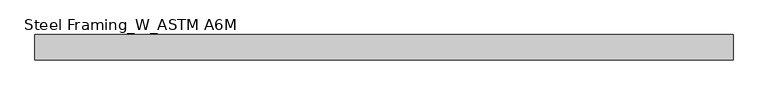
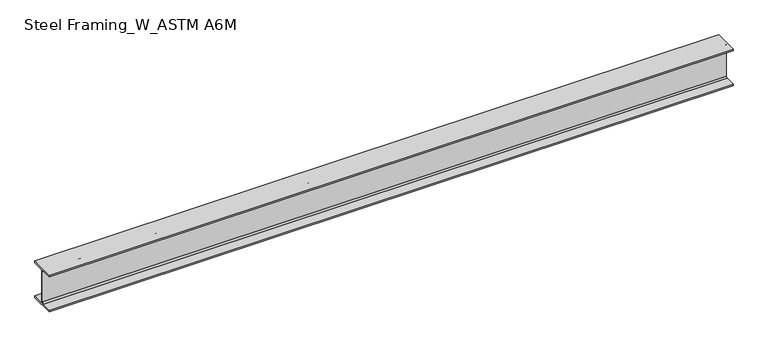
"""IFC4 building model written with IfcOpenShell, lengths in millimetres: beam geometry, Steel Framing_W_ASTM A6M : H_SB_AR_S02_W200x31.3_B6."""

from ifc_helpers import new_model, si_unit, point, frame, frame_2d, origin, place, context, project, spatial, polyline, circle_curve, trimmed, segment, composite_curve, outline, extrude, source, transform, mapped, element, save


def steel_framing_w_astm_a6m_5d0dfb1e(model_context):
    return source(origin(), model_context, "Body", "SweptSolid", [
        extrude(outline(composite_curve([segment(polyline([(67.0, -94.8), (67.0, -105.0), (-67.0, -105.0), (-67.0, -94.8), (-10.775, -94.8)]), True, "CONTINUOUS"), segment(trimmed(circle_curve(frame_2d((-10.775, -87.2)), 7.6), [point((-10.775, -94.8))], [point((-3.175, -87.2))], True, "CARTESIAN"), True, "CONTINUOUS"), segment(polyline([(-3.175, -87.2), (-3.175, 87.2)]), True, "CONTINUOUS"), segment(trimmed(circle_curve(frame_2d((-10.775, 87.2)), 7.6), [point((-3.175, 87.2))], [point((-10.775, 94.8))], True, "CARTESIAN"), True, "CONTINUOUS"), segment(polyline([(-10.775, 94.8), (-67.0, 94.8), (-67.0, 105.0), (67.0, 105.0), (67.0, 94.8), (10.775, 94.8)]), True, "CONTINUOUS"), segment(trimmed(circle_curve(frame_2d((10.775, 87.2)), 7.6), [point((10.775, 94.8))], [point((3.175, 87.2))], True, "CARTESIAN"), True, "CONTINUOUS"), segment(polyline([(3.175, 87.2), (3.175, -87.2)]), True, "CONTINUOUS"), segment(trimmed(circle_curve(frame_2d((10.775, -87.2)), 7.6), [point((3.175, -87.2))], [point((10.775, -94.8))], True, "CARTESIAN"), True, "CONTINUOUS"), segment(polyline([(10.775, -94.8), (67.0, -94.8)]), True, "CONTINUOUS")], self_intersect=False)), frame((-1846.3, 0.0, 0.0), z_axis=(1.0, 0.0, 0.0), x_axis=(0.0, 1.0, 0.0)), (0.0, 0.0, 1.0), 3692.6),
    ])


if __name__ == "__main__":
    model = new_model("IFC4")
    model_context = context("Model", 3, world=origin())
    ifc_project = project(units=[si_unit("LENGTHUNIT", "METRE", prefix="MILLI")], contexts=[model_context])
    site = spatial("IfcSite", under=ifc_project)
    building = spatial("IfcBuilding", under=site)
    placement = place(None, origin())
    steel_framing_w_astm_a6m_shape = steel_framing_w_astm_a6m_5d0dfb1e(model_context)
    element("IfcBeam", 1, ObjectType="Steel Framing_W_ASTM A6M : H_SB_AR_S02_W200x31.3_B6", at=placement, inside=building, context=model_context, shape_type="MappedRepresentation", body=[
        mapped(steel_framing_w_astm_a6m_shape, transform((0.0, 0.0, 0.0), x_axis=(1.0, 0.0, 0.0), y_axis=(0.0, 1.0, 0.0), z_axis=(0.0, 0.0, 1.0))),
    ])
    save(model, "model.ifc")

# Revit data of these elements
# Type "Steel Framing_W_ASTM A6M : H_SB_AR_S02_W200x31.3_B6"
#   Type Mark = "B6"
#   Section Name Key = "W8x21"
#   Width = 13.4 cm
#   Web Thickness = 0.635 cm
#   Web Fillet = 0.76 cm
#   Warping Constant = 40800.0 cm⁶
#   Torsional Moment of Inertia = 11.70 cm⁴
#   Section Area = 39.7 cm²
#   Plastic Modulus weak axis = 93.2 cm³
#   Plastic Modulus strong axis = 334.0 cm³
#   Perimeter = 0.93 m²/m
#   Nominal Weight = 31.30 kgf/m
#   Moment of Inertia weak axis = 407.00 cm⁴
#   Moment of Inertia strong axis = 3130.00 cm⁴
#   Height = 21.0 cm
#   Flange Thickness = 1.02 cm
#   Elastic Modulus weak axis = 60.8 cm³
#   Elastic Modulus strong axis = 298.0 cm³
#   Centroid Vertical = 10.5 cm
#   Centroid Horizontal = 6.7 cm
#   Length [instance default] = 1500 mm
#   Structural Material [instance default] = Steel, 45-345
#   Bolt Spacing = 0
#   Assembly Code = ""
# Element 1 (IfcBeam, "Steel Framing_W_ASTM A6M : H_SB_AR_S02_W200x31.3_B6")
#   Materials on its faces: "Steel, 45-345"
# Materials
#   "Steel, 45-345": class "Metal", colour RGB 189 187 185, transparency 0, Description = "Steel 345 MPa", Cost = 0
